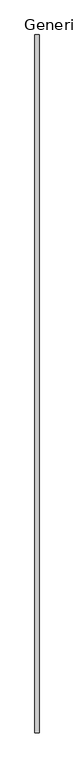
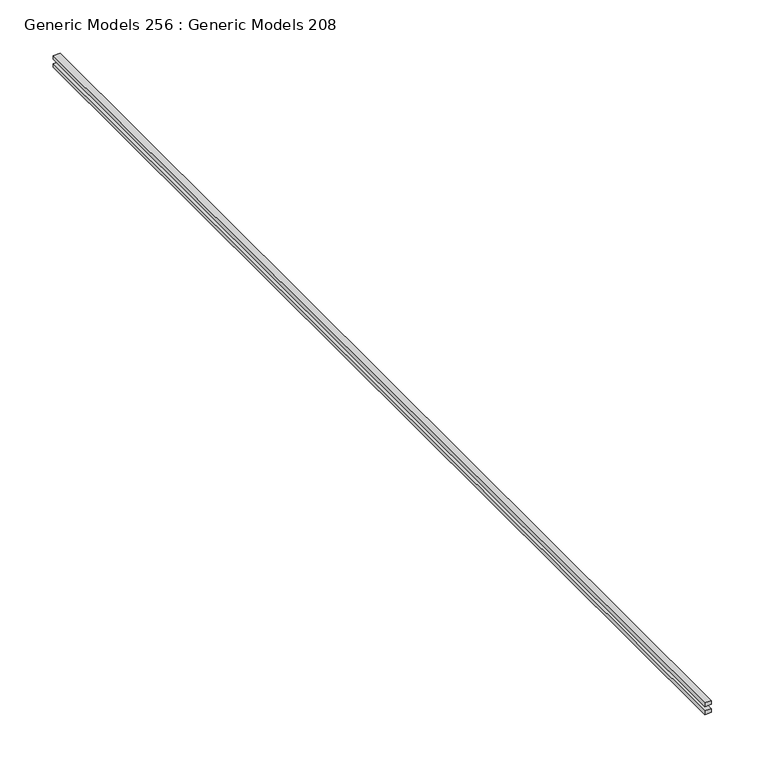
"""IFC4 building model written with IfcOpenShell, lengths in millimetres: proxy geometry, Generic Models 256 : Generic Models 208."""

from ifc_helpers import new_model, si_unit, frame, origin, place, context, project, spatial, polyline, outline, extrude, source, transform, mapped, element, save


def generic_models_256_generic_models_208_ebb3bc28(model_context):
    return source(origin(), model_context, "Body", "SweptSolid", [
        extrude(outline(polyline([(53726.4135017, 990.4966182), (53733.5579225, 990.4966182), (53733.5579225, -228.7033818), (53726.4135017, -228.7033818), (53726.4135017, 990.4966182)])), frame((0.0, 0.0, 2042.0815912), z_axis=(0.0, 0.0, 1.0), x_axis=(1.0, 0.0, 0.0)), (0.0, 0.0, 1.0), 4.2333333),
        extrude(outline(polyline([(53726.4135017, 990.4966182), (53733.5579225, 990.4966182), (53733.5579225, -228.7033818), (53726.4135017, -228.7033818), (53726.4135017, 990.4966182)])), frame((0.0, 0.0, 2033.0857579), z_axis=(0.0, 0.0, 1.0), x_axis=(1.0, 0.0, 0.0)), (0.0, 0.0, 1.0), 4.2333333),
    ])


if __name__ == "__main__":
    model = new_model("IFC4")
    model_context = context("Model", 3, world=origin())
    ifc_project = project(units=[si_unit("LENGTHUNIT", "METRE", prefix="MILLI")], contexts=[model_context])
    site = spatial("IfcSite", under=ifc_project)
    building = spatial("IfcBuilding", under=site)
    placement = place(None, origin())
    generic_models_256_generic_models_208_shape = generic_models_256_generic_models_208_ebb3bc28(model_context)
    element("IfcBuildingElementProxy", 1, Name="Generic Models 256 : Generic Models 208", ObjectType="Generic Models 256 : Generic Models 208", at=placement, inside=building, context=model_context, shape_type="MappedRepresentation", body=[
        mapped(generic_models_256_generic_models_208_shape, transform((0.0, 0.0, 0.0), x_axis=(1.0, 0.0, 0.0), y_axis=(0.0, 1.0, 0.0), z_axis=(0.0, 0.0, 1.0))),
    ])
    save(model, "model.ifc")

# Revit data of these elements
# Element 1 (IfcBuildingElementProxy, "Generic Models 256 : Generic Models 208")
#   Materials on its faces: "UNISTRUT 1/4\" FIBERGLASS HEX FLANGED BOLT"
# Materials
#   "UNISTRUT 1/4\" FIBERGLASS HEX FLANGED BOLT": class "Miscellaneous", colour RGB 236 232 217, transparency 0, Cost = 0
